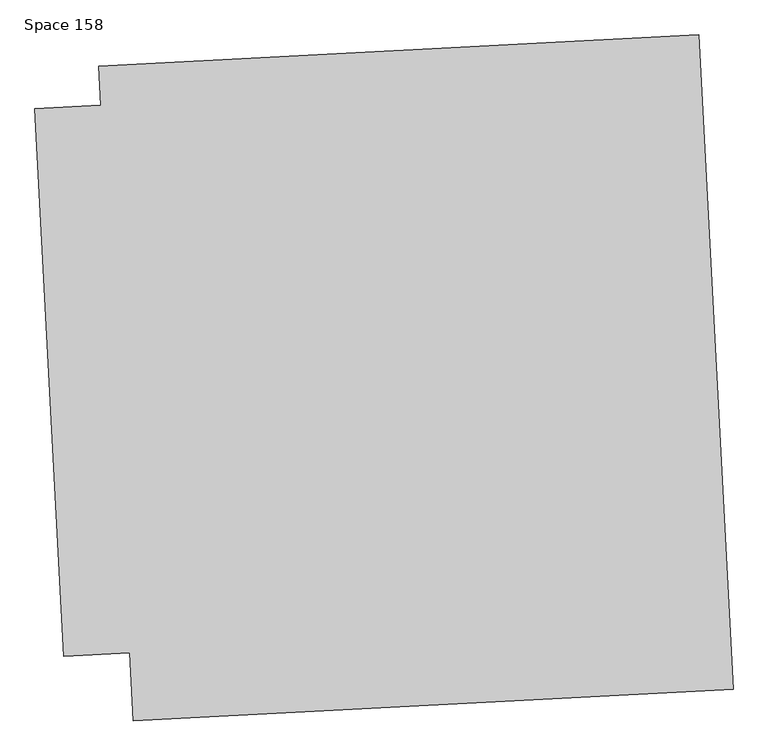
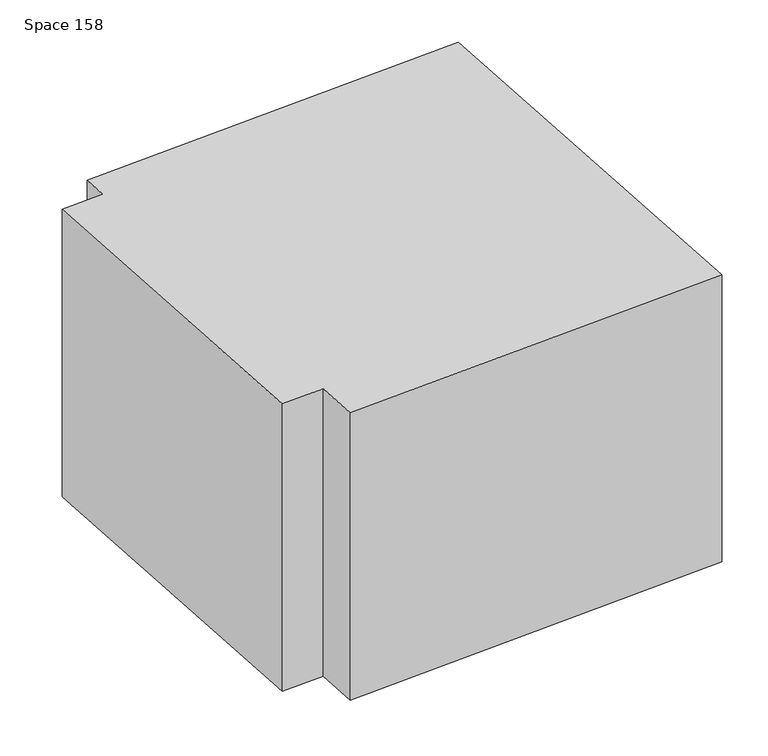
"""IFC4 building model written with IfcOpenShell, lengths in millimetres: proxy geometry, Space 158."""

from ifc_helpers import new_model, si_unit, frame, origin, place, context, project, spatial, polyline, outline, extrude, source, transform, mapped, element, save


def space_158_16205067(model_context):
    return source(origin(), model_context, "Body", "SweptSolid", [
        extrude(outline(polyline([(-10240.1651681, -31941.5237784), (-9818.4688813, -31919.4236125), (-9831.5960475, -31668.9423595), (-5991.9403836, -31467.7145329), (-5772.2680577, -35659.3122106), (-9611.9237216, -35860.5400372), (-9634.6885541, -35426.1611553), (-10056.3848409, -35448.2613212), (-10240.1651681, -31941.5237784)])), frame((0.0, 0.0, 3810.0), z_axis=(0.0, 0.0, 1.0), x_axis=(1.0, 0.0, 0.0)), (0.0, 0.0, 1.0), 3048.0),
    ])


if __name__ == "__main__":
    model = new_model("IFC4")
    model_context = context("Model", 3, world=origin())
    ifc_project = project(units=[si_unit("LENGTHUNIT", "METRE", prefix="MILLI")], contexts=[model_context])
    site = spatial("IfcSite", under=ifc_project)
    building = spatial("IfcBuilding", under=site)
    placement = place(None, origin())
    space_158_shape = space_158_16205067(model_context)
    element("IfcBuildingElementProxy", 1, Name="Space 158", ObjectType="Space 158", at=placement, inside=building, context=model_context, shape_type="MappedRepresentation", body=[
        mapped(space_158_shape, transform((0.0, 0.0, 0.0), x_axis=(1.0, 0.0, 0.0), y_axis=(0.0, 1.0, 0.0), z_axis=(0.0, 0.0, 1.0))),
    ])
    save(model, "model.ifc")

# Revit data of these elements
# Element 1 (IfcBuildingElementProxy, "Space 158")
#   Materials on its faces: "Render Material 255-255-255"
# Materials
#   "Render Material 255-255-255": class "Unassigned", colour RGB 255 255 255, transparency 0
